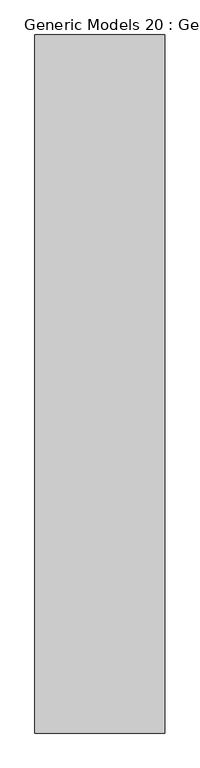
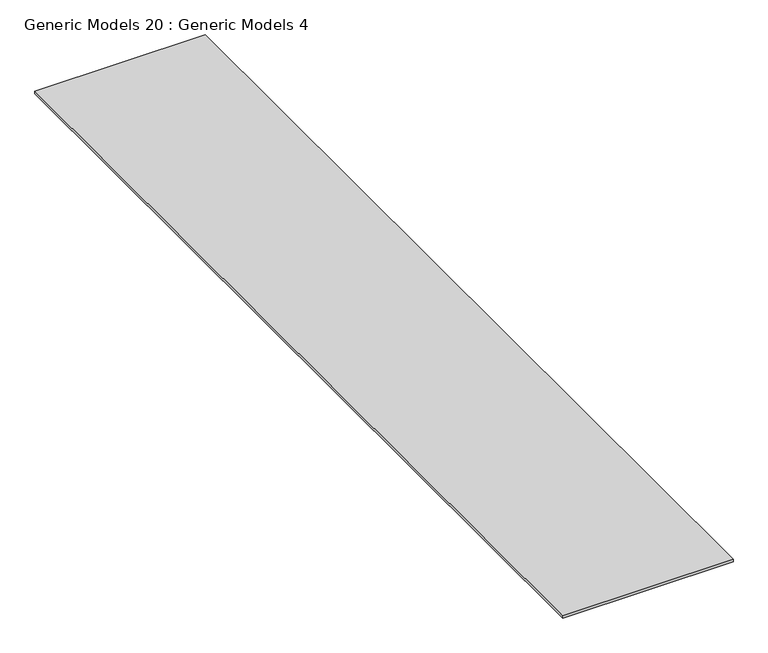
"""IFC4 building model written with IfcOpenShell, lengths in millimetres: proxy geometry, Generic Models 20 : Generic Models 4."""

from ifc_helpers import new_model, si_unit, frame, origin, place, context, project, spatial, polyline, outline, extrude, source, transform, mapped, element, save


def generic_models_20_generic_models_4_02edee59(model_context):
    return source(origin(), model_context, "Body", "SweptSolid", [
        extrude(outline(polyline([(-8369.4736296, 7054.2769662), (-9249.2270433, 7054.2769662), (-9249.2270433, 11778.6769662), (-8369.4736296, 11778.6769662), (-8369.4736296, 7054.2769662)])), frame((0.0, 0.0, 126380.6425653), z_axis=(0.0, 0.0, 1.0), x_axis=(1.0, 0.0, 0.0)), (0.0, 0.0, 1.0), 12.7),
    ])


if __name__ == "__main__":
    model = new_model("IFC4")
    model_context = context("Model", 3, world=origin())
    ifc_project = project(units=[si_unit("LENGTHUNIT", "METRE", prefix="MILLI")], contexts=[model_context])
    site = spatial("IfcSite", under=ifc_project)
    building = spatial("IfcBuilding", under=site)
    placement = place(None, origin())
    generic_models_20_generic_models_4_shape = generic_models_20_generic_models_4_02edee59(model_context)
    element("IfcBuildingElementProxy", 1, Name="Generic Models 20 : Generic Models 4", ObjectType="Generic Models 20 : Generic Models 4", at=placement, inside=building, context=model_context, shape_type="MappedRepresentation", body=[
        mapped(generic_models_20_generic_models_4_shape, transform((0.0, 0.0, 0.0), x_axis=(1.0, 0.0, 0.0), y_axis=(0.0, 1.0, 0.0), z_axis=(0.0, 0.0, 1.0))),
    ])
    save(model, "model.ifc")

# Revit data of these elements
# Element 1 (IfcBuildingElementProxy, "Generic Models 20 : Generic Models 4")
#   Materials on its faces: "_1/2\" CDX PLYWOOD"
# Materials
#   "_1/2\" CDX PLYWOOD": class "Generic", colour RGB 98 75 74, transparency 0, Cost = 0
